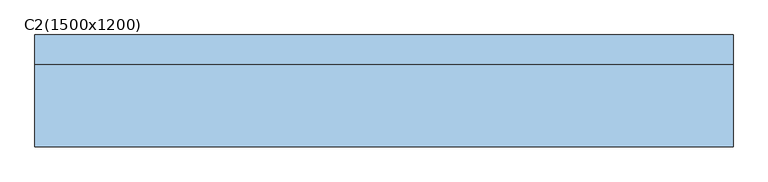
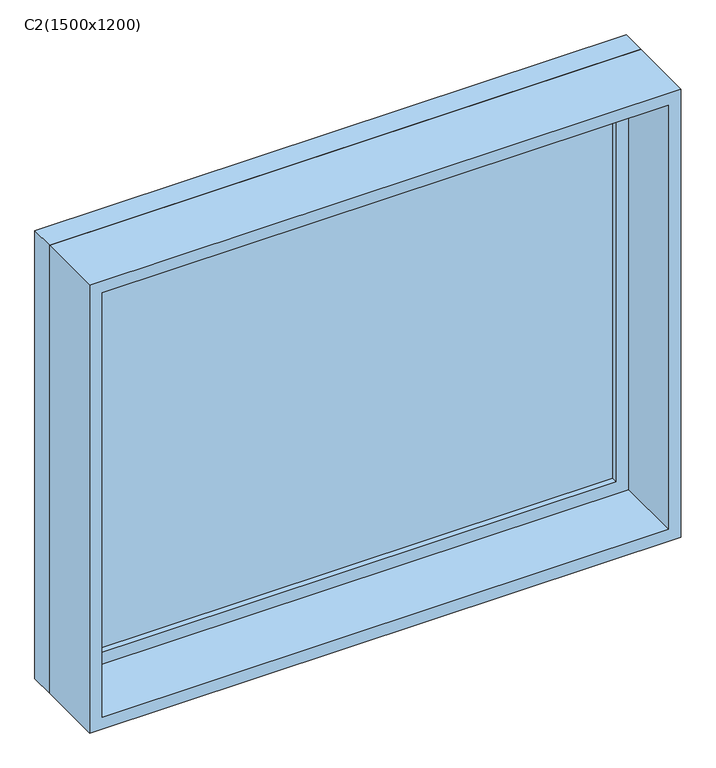
"""IFC4 building model written with IfcOpenShell, lengths in millimetres: window geometry, 固定窗 : C2(1500x1200)."""

from ifc_helpers import new_model, si_unit, frame, origin, place, context, project, spatial, polyline, outline, extrude, source, transform, mapped, element, save


def c2_1500x1200_cfff0f4c(model_context):
    return source(origin(), model_context, "Body", "SweptSolid", [
        extrude(outline(polyline([(648.4, 71.425), (-724.6, 71.425), (-724.6, 84.125), (648.4, 84.125), (648.4, 71.425)])), frame((0.0, 0.0, 963.5), z_axis=(0.0, 0.0, 1.0), x_axis=(1.0, 0.0, 0.0)), (0.0, 0.0, 1.0), 1073.0),
        extrude(outline(polyline([(2080.95, -769.05), (919.05, -769.05), (919.05, 692.85), (2080.95, 692.85), (2080.95, -769.05)]), holes=[polyline([(2036.5, -724.6), (2036.5, 648.4), (963.5, 648.4), (963.5, -724.6), (2036.5, -724.6)])]), frame((0.0, 55.55, 0.0), z_axis=(0.0, 1.0, 0.0), x_axis=(0.0, 0.0, 1.0)), (0.0, 0.0, 1.0), 44.45),
        extrude(outline(polyline([(2100.0, -788.1), (900.0, -788.1), (900.0, 711.9), (2100.0, 711.9), (2100.0, -788.1)]), holes=[polyline([(2068.25, -756.35), (2068.25, 680.15), (931.75, 680.15), (931.75, -756.35), (2068.25, -756.35)])]), frame((0.0, -120.0, 0.0), z_axis=(0.0, 1.0, 0.0), x_axis=(0.0, 0.0, 1.0)), (0.0, 0.0, 1.0), 175.55),
        extrude(outline(polyline([(2100.0, 711.9), (2100.0, -788.1), (900.0, -788.1), (900.0, 711.9), (2100.0, 711.9)]), holes=[polyline([(2080.95, 692.85), (919.05, 692.85), (919.05, -769.05), (2080.95, -769.05), (2080.95, 692.85)])]), frame((0.0, 55.55, 0.0), z_axis=(0.0, 1.0, 0.0), x_axis=(0.0, 0.0, 1.0)), (0.0, 0.0, 1.0), 64.45),
    ])


if __name__ == "__main__":
    model = new_model("IFC4")
    model_context = context("Model", 3, world=origin())
    ifc_project = project(units=[si_unit("LENGTHUNIT", "METRE", prefix="MILLI")], contexts=[model_context])
    site = spatial("IfcSite", under=ifc_project)
    building = spatial("IfcBuilding", under=site)
    placement = place(None, origin())
    c2_1500x1200_shape = c2_1500x1200_cfff0f4c(model_context)
    element("IfcWindow", 1, ObjectType="固定窗 : C2(1500x1200)", at=placement, inside=building, context=model_context, shape_type="MappedRepresentation", body=[
        mapped(c2_1500x1200_shape, transform((0.0, 0.0, 0.0), x_axis=(1.0, 0.0, 0.0), y_axis=(0.0, 1.0, 0.0), z_axis=(0.0, 0.0, 1.0))),
    ])
    save(model, "model.ifc")

# Revit data of these elements
# Type "固定窗 : C2(1500x1200)"
#   Type Mark = "C1517"
#   Construction Type Id = "SGL"
#   Analytic Construction = "大型单层玻璃窗"
#   Visual Light Transmittance = 0.9
#   Solar Heat Gain Coefficient = 0.86
#   Rough Width = 1500 mm
#   Rough Height = 1200 mm
#   Heat Transfer Coefficient (U) = 5.5617 W/(m²·K)
#   Height = 1200 mm
#   默认窗台高度 = 900 mm
#   Width = 1500 mm
#   窗嵌入 = 20 mm
#   高窗平面 [instance default] = no
#   通用窗平面 [instance default] = yes
#   玻璃 = none
#   框架材质 = none
#   Wall Closure = (empty or 0)
# Element 1 (IfcWindow, "固定窗 : C2(1500x1200)")
#   Materials on its faces: "玻璃"
# Materials
#   "玻璃": class "玻璃", colour RGB 0 128 192, transparency 0.9, Description = "钠钙玻璃", Cost = 0
